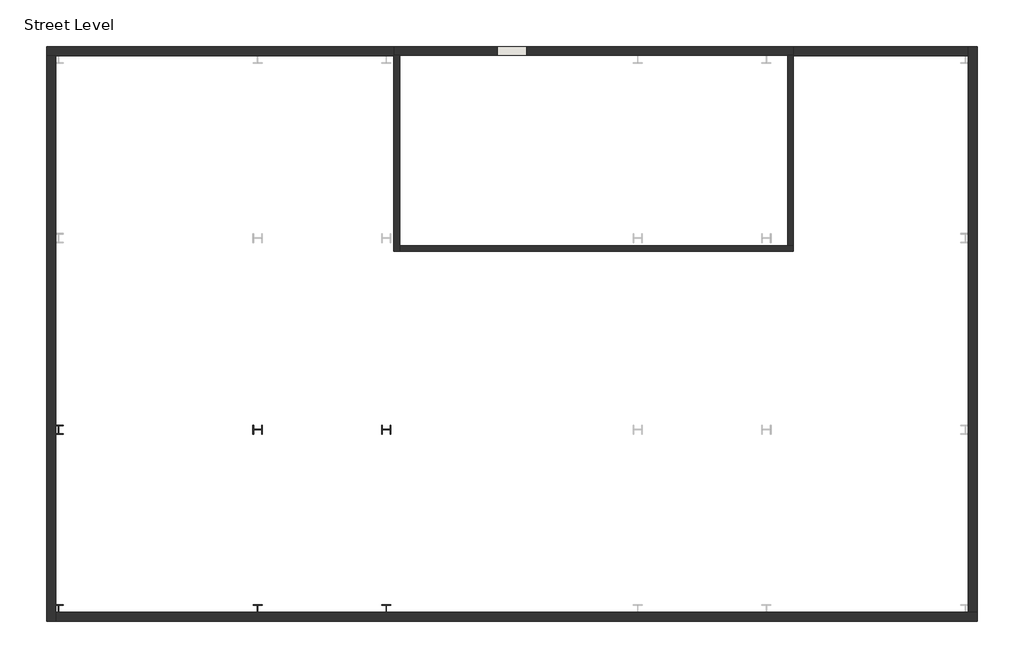
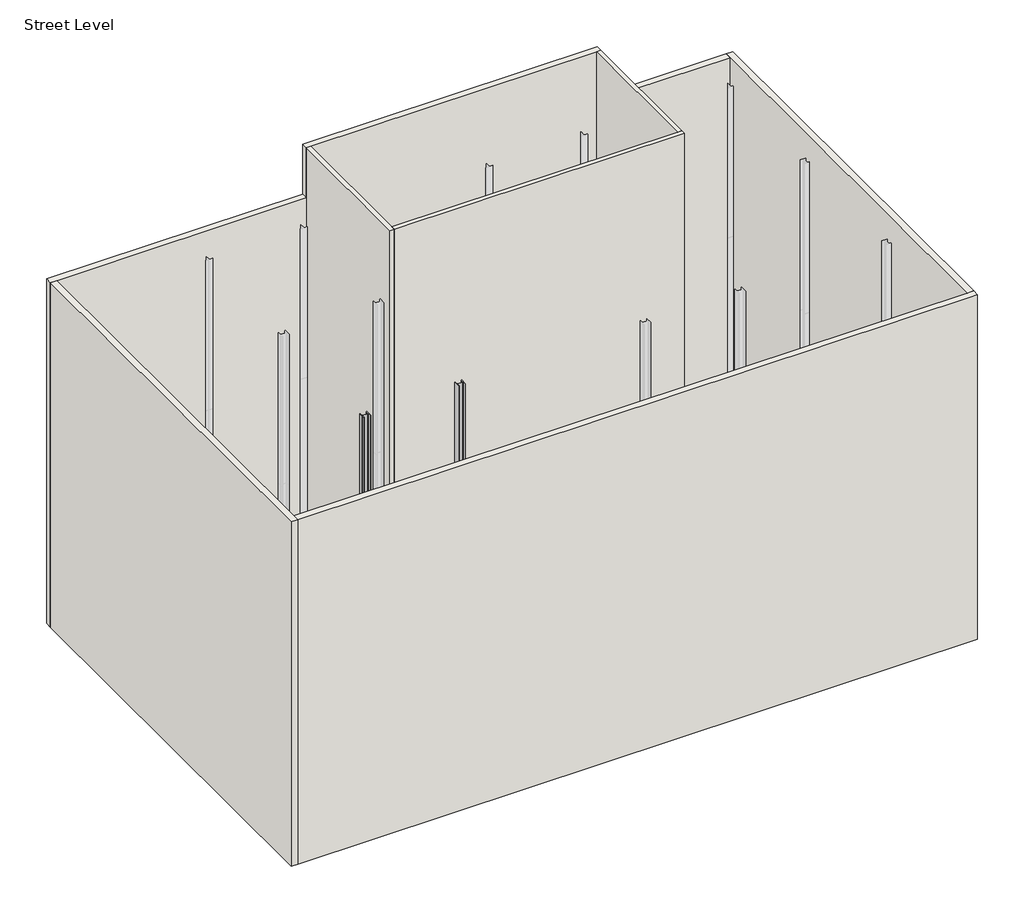
# One storey, part 1 of 3: 9 walls, 6 columns.
"""IFC4 building model written with IfcOpenShell, lengths in millimetres."""

from ifc_helpers import new_model, si_unit, point, frame, frame_2d, origin, place, context, project, spatial, polyline, circle_curve, trimmed, segment, composite_curve, outline, extrude, faceted_brep, element, save

model = new_model("IFC4")

# Units and contexts
model_context = context("Model", 3, world=origin())
ifc_project = project(units=[si_unit("LENGTHUNIT", "METRE", prefix="MILLI")], contexts=[model_context])

# Site, building, storey
site = spatial("IfcSite", under=ifc_project)
building = spatial("IfcBuilding", under=site)
storey = spatial("IfcBuildingStorey", under=building, Name="Street Level", Elevation=-914.4)

# Columns
placement = place(None, origin())
element("IfcColumn", 1, ObjectType="W-Wide Flange-Column : W12X87", at=placement, inside=storey, context=model_context, shape_type="SweptSolid", body=[
    extrude(outline(composite_curve([segment(polyline([(-9643.0622732, -3562.1684696), (-9663.6362732, -3562.1684696), (-9663.6362732, -3437.3274696)]), True, "CONTINUOUS"), segment(trimmed(circle_curve(frame_2d((-9685.9247732, -3437.3274696)), 22.2885), [point((-9663.6362732, -3437.3274696))], [point((-9685.9247732, -3415.0389696))], True, "CARTESIAN"), True, "CONTINUOUS"), segment(polyline([(-9685.9247732, -3415.0389696), (-9917.6997732, -3415.0389696)]), True, "CONTINUOUS"), segment(trimmed(circle_curve(frame_2d((-9917.6997732, -3437.3274696)), 22.2885), [point((-9917.6997732, -3415.0389696))], [point((-9939.9882732, -3437.3274696))], True, "CARTESIAN"), True, "CONTINUOUS"), segment(polyline([(-9939.9882732, -3437.3274696), (-9939.9882732, -3562.1684696), (-9960.5622732, -3562.1684696), (-9960.5622732, -3254.8284696), (-9939.9882732, -3254.8284696), (-9939.9882732, -3379.6694696)]), True, "CONTINUOUS"), segment(trimmed(circle_curve(frame_2d((-9917.6997732, -3379.6694696)), 22.2885), [point((-9939.9882732, -3379.6694696))], [point((-9917.6997732, -3401.9579696))], True, "CARTESIAN"), True, "CONTINUOUS"), segment(polyline([(-9917.6997732, -3401.9579696), (-9685.9247732, -3401.9579696)]), True, "CONTINUOUS"), segment(trimmed(circle_curve(frame_2d((-9685.9247732, -3379.6694696)), 22.2885), [point((-9685.9247732, -3401.9579696))], [point((-9663.6362732, -3379.6694696))], True, "CARTESIAN"), True, "CONTINUOUS"), segment(polyline([(-9663.6362732, -3379.6694696), (-9663.6362732, -3254.8284696), (-9643.0622732, -3254.8284696), (-9643.0622732, -3562.1684696)]), True, "CONTINUOUS")], self_intersect=False)), frame((0.0, 0.0, 7315.2), z_axis=(0.0, 0.0, 1.0), x_axis=(1.0, 0.0, 0.0)), (0.0, 0.0, 1.0), 7315.2),
    extrude(outline(composite_curve([segment(polyline([(-9643.0622732, -3562.1684696), (-9663.6362732, -3562.1684696), (-9663.6362732, -3437.3274696)]), True, "CONTINUOUS"), segment(trimmed(circle_curve(frame_2d((-9685.9247732, -3437.3274696)), 22.2885), [point((-9663.6362732, -3437.3274696))], [point((-9685.9247732, -3415.0389696))], True, "CARTESIAN"), True, "CONTINUOUS"), segment(polyline([(-9685.9247732, -3415.0389696), (-9917.6997732, -3415.0389696)]), True, "CONTINUOUS"), segment(trimmed(circle_curve(frame_2d((-9917.6997732, -3437.3274696)), 22.2885), [point((-9917.6997732, -3415.0389696))], [point((-9939.9882732, -3437.3274696))], True, "CARTESIAN"), True, "CONTINUOUS"), segment(polyline([(-9939.9882732, -3437.3274696), (-9939.9882732, -3562.1684696), (-9960.5622732, -3562.1684696), (-9960.5622732, -3254.8284696), (-9939.9882732, -3254.8284696), (-9939.9882732, -3379.6694696)]), True, "CONTINUOUS"), segment(trimmed(circle_curve(frame_2d((-9917.6997732, -3379.6694696)), 22.2885), [point((-9939.9882732, -3379.6694696))], [point((-9917.6997732, -3401.9579696))], True, "CARTESIAN"), True, "CONTINUOUS"), segment(polyline([(-9917.6997732, -3401.9579696), (-9685.9247732, -3401.9579696)]), True, "CONTINUOUS"), segment(trimmed(circle_curve(frame_2d((-9685.9247732, -3379.6694696)), 22.2885), [point((-9685.9247732, -3401.9579696))], [point((-9663.6362732, -3379.6694696))], True, "CARTESIAN"), True, "CONTINUOUS"), segment(polyline([(-9663.6362732, -3379.6694696), (-9663.6362732, -3254.8284696), (-9643.0622732, -3254.8284696), (-9643.0622732, -3562.1684696)]), True, "CONTINUOUS")], self_intersect=False)), frame((0.0, 0.0, -914.4), z_axis=(0.0, 0.0, 1.0), x_axis=(1.0, 0.0, 0.0)), (0.0, 0.0, 1.0), 8229.6),
])
element("IfcColumn", 2, ObjectType="W-Wide Flange-Column : W12X87", at=placement, inside=storey, context=model_context, shape_type="SweptSolid", body=[
    extrude(outline(composite_curve([segment(polyline([(-5274.2622732, -3562.1684696), (-5294.8362732, -3562.1684696), (-5294.8362732, -3437.3274696)]), True, "CONTINUOUS"), segment(trimmed(circle_curve(frame_2d((-5317.1247732, -3437.3274696)), 22.2885), [point((-5294.8362732, -3437.3274696))], [point((-5317.1247732, -3415.0389696))], True, "CARTESIAN"), True, "CONTINUOUS"), segment(polyline([(-5317.1247732, -3415.0389696), (-5548.8997732, -3415.0389696)]), True, "CONTINUOUS"), segment(trimmed(circle_curve(frame_2d((-5548.8997732, -3437.3274696)), 22.2885), [point((-5548.8997732, -3415.0389696))], [point((-5571.1882732, -3437.3274696))], True, "CARTESIAN"), True, "CONTINUOUS"), segment(polyline([(-5571.1882732, -3437.3274696), (-5571.1882732, -3562.1684696), (-5591.7622732, -3562.1684696), (-5591.7622732, -3254.8284696), (-5571.1882732, -3254.8284696), (-5571.1882732, -3379.6694696)]), True, "CONTINUOUS"), segment(trimmed(circle_curve(frame_2d((-5548.8997732, -3379.6694696)), 22.2885), [point((-5571.1882732, -3379.6694696))], [point((-5548.8997732, -3401.9579696))], True, "CARTESIAN"), True, "CONTINUOUS"), segment(polyline([(-5548.8997732, -3401.9579696), (-5317.1247732, -3401.9579696)]), True, "CONTINUOUS"), segment(trimmed(circle_curve(frame_2d((-5317.1247732, -3379.6694696)), 22.2885), [point((-5317.1247732, -3401.9579696))], [point((-5294.8362732, -3379.6694696))], True, "CARTESIAN"), True, "CONTINUOUS"), segment(polyline([(-5294.8362732, -3379.6694696), (-5294.8362732, -3254.8284696), (-5274.2622732, -3254.8284696), (-5274.2622732, -3562.1684696)]), True, "CONTINUOUS")], self_intersect=False)), frame((0.0, 0.0, 7315.2), z_axis=(0.0, 0.0, 1.0), x_axis=(1.0, 0.0, 0.0)), (0.0, 0.0, 1.0), 7315.2),
    extrude(outline(composite_curve([segment(polyline([(-5274.2622732, -3562.1684696), (-5294.8362732, -3562.1684696), (-5294.8362732, -3437.3274696)]), True, "CONTINUOUS"), segment(trimmed(circle_curve(frame_2d((-5317.1247732, -3437.3274696)), 22.2885), [point((-5294.8362732, -3437.3274696))], [point((-5317.1247732, -3415.0389696))], True, "CARTESIAN"), True, "CONTINUOUS"), segment(polyline([(-5317.1247732, -3415.0389696), (-5548.8997732, -3415.0389696)]), True, "CONTINUOUS"), segment(trimmed(circle_curve(frame_2d((-5548.8997732, -3437.3274696)), 22.2885), [point((-5548.8997732, -3415.0389696))], [point((-5571.1882732, -3437.3274696))], True, "CARTESIAN"), True, "CONTINUOUS"), segment(polyline([(-5571.1882732, -3437.3274696), (-5571.1882732, -3562.1684696), (-5591.7622732, -3562.1684696), (-5591.7622732, -3254.8284696), (-5571.1882732, -3254.8284696), (-5571.1882732, -3379.6694696)]), True, "CONTINUOUS"), segment(trimmed(circle_curve(frame_2d((-5548.8997732, -3379.6694696)), 22.2885), [point((-5571.1882732, -3379.6694696))], [point((-5548.8997732, -3401.9579696))], True, "CARTESIAN"), True, "CONTINUOUS"), segment(polyline([(-5548.8997732, -3401.9579696), (-5317.1247732, -3401.9579696)]), True, "CONTINUOUS"), segment(trimmed(circle_curve(frame_2d((-5317.1247732, -3379.6694696)), 22.2885), [point((-5317.1247732, -3401.9579696))], [point((-5294.8362732, -3379.6694696))], True, "CARTESIAN"), True, "CONTINUOUS"), segment(polyline([(-5294.8362732, -3379.6694696), (-5294.8362732, -3254.8284696), (-5274.2622732, -3254.8284696), (-5274.2622732, -3562.1684696)]), True, "CONTINUOUS")], self_intersect=False)), frame((0.0, 0.0, -914.4), z_axis=(0.0, 0.0, 1.0), x_axis=(1.0, 0.0, 0.0)), (0.0, 0.0, 1.0), 8229.6),
])
element("IfcColumn", 3, ObjectType="W-Wide Flange-Column : W12X87", at=placement, inside=storey, context=model_context, shape_type="SweptSolid", body=[
    extrude(outline(composite_curve([segment(polyline([(-5279.3422732, -9345.7484696), (-5279.3422732, -9366.3224696), (-5404.1832732, -9366.3224696)]), True, "CONTINUOUS"), segment(trimmed(circle_curve(frame_2d((-5404.1832732, -9388.6109696)), 22.2885), [point((-5404.1832732, -9366.3224696))], [point((-5426.4717732, -9388.6109696))], True, "CARTESIAN"), True, "CONTINUOUS"), segment(polyline([(-5426.4717732, -9388.6109696), (-5426.4717732, -9620.3859696)]), True, "CONTINUOUS"), segment(trimmed(circle_curve(frame_2d((-5404.1832732, -9620.3859696)), 22.2885), [point((-5426.4717732, -9620.3859696))], [point((-5404.1832732, -9642.6744696))], True, "CARTESIAN"), True, "CONTINUOUS"), segment(polyline([(-5404.1832732, -9642.6744696), (-5279.3422732, -9642.6744696), (-5279.3422732, -9663.2484696), (-5586.6822732, -9663.2484696), (-5586.6822732, -9642.6744696), (-5461.8412732, -9642.6744696)]), True, "CONTINUOUS"), segment(trimmed(circle_curve(frame_2d((-5461.8412732, -9620.3859696)), 22.2885), [point((-5461.8412732, -9642.6744696))], [point((-5439.5527732, -9620.3859696))], True, "CARTESIAN"), True, "CONTINUOUS"), segment(polyline([(-5439.5527732, -9620.3859696), (-5439.5527732, -9388.6109696)]), True, "CONTINUOUS"), segment(trimmed(circle_curve(frame_2d((-5461.8412732, -9388.6109696)), 22.2885), [point((-5439.5527732, -9388.6109696))], [point((-5461.8412732, -9366.3224696))], True, "CARTESIAN"), True, "CONTINUOUS"), segment(polyline([(-5461.8412732, -9366.3224696), (-5586.6822732, -9366.3224696), (-5586.6822732, -9345.7484696), (-5279.3422732, -9345.7484696)]), True, "CONTINUOUS")], self_intersect=False)), frame((0.0, 0.0, 7315.2), z_axis=(0.0, 0.0, 1.0), x_axis=(1.0, 0.0, 0.0)), (0.0, 0.0, 1.0), 7315.2),
    extrude(outline(composite_curve([segment(polyline([(-5279.3422732, -9345.7484696), (-5279.3422732, -9366.3224696), (-5404.1832732, -9366.3224696)]), True, "CONTINUOUS"), segment(trimmed(circle_curve(frame_2d((-5404.1832732, -9388.6109696)), 22.2885), [point((-5404.1832732, -9366.3224696))], [point((-5426.4717732, -9388.6109696))], True, "CARTESIAN"), True, "CONTINUOUS"), segment(polyline([(-5426.4717732, -9388.6109696), (-5426.4717732, -9620.3859696)]), True, "CONTINUOUS"), segment(trimmed(circle_curve(frame_2d((-5404.1832732, -9620.3859696)), 22.2885), [point((-5426.4717732, -9620.3859696))], [point((-5404.1832732, -9642.6744696))], True, "CARTESIAN"), True, "CONTINUOUS"), segment(polyline([(-5404.1832732, -9642.6744696), (-5279.3422732, -9642.6744696), (-5279.3422732, -9663.2484696), (-5586.6822732, -9663.2484696), (-5586.6822732, -9642.6744696), (-5461.8412732, -9642.6744696)]), True, "CONTINUOUS"), segment(trimmed(circle_curve(frame_2d((-5461.8412732, -9620.3859696)), 22.2885), [point((-5461.8412732, -9642.6744696))], [point((-5439.5527732, -9620.3859696))], True, "CARTESIAN"), True, "CONTINUOUS"), segment(polyline([(-5439.5527732, -9620.3859696), (-5439.5527732, -9388.6109696)]), True, "CONTINUOUS"), segment(trimmed(circle_curve(frame_2d((-5461.8412732, -9388.6109696)), 22.2885), [point((-5439.5527732, -9388.6109696))], [point((-5461.8412732, -9366.3224696))], True, "CARTESIAN"), True, "CONTINUOUS"), segment(polyline([(-5461.8412732, -9366.3224696), (-5586.6822732, -9366.3224696), (-5586.6822732, -9345.7484696), (-5279.3422732, -9345.7484696)]), True, "CONTINUOUS")], self_intersect=False)), frame((0.0, 0.0, -914.4), z_axis=(0.0, 0.0, 1.0), x_axis=(1.0, 0.0, 0.0)), (0.0, 0.0, 1.0), 8229.6),
])
element("IfcColumn", 4, ObjectType="W-Wide Flange-Column : W12X87", at=placement, inside=storey, context=model_context, shape_type="SweptSolid", body=[
    extrude(outline(composite_curve([segment(polyline([(-9648.1422732, -9345.7484696), (-9648.1422732, -9366.3224696), (-9772.9832732, -9366.3224696)]), True, "CONTINUOUS"), segment(trimmed(circle_curve(frame_2d((-9772.9832732, -9388.6109696)), 22.2885), [point((-9772.9832732, -9366.3224696))], [point((-9795.2717732, -9388.6109696))], True, "CARTESIAN"), True, "CONTINUOUS"), segment(polyline([(-9795.2717732, -9388.6109696), (-9795.2717732, -9620.3859696)]), True, "CONTINUOUS"), segment(trimmed(circle_curve(frame_2d((-9772.9832732, -9620.3859696)), 22.2885), [point((-9795.2717732, -9620.3859696))], [point((-9772.9832732, -9642.6744696))], True, "CARTESIAN"), True, "CONTINUOUS"), segment(polyline([(-9772.9832732, -9642.6744696), (-9648.1422732, -9642.6744696), (-9648.1422732, -9663.2484696), (-9955.4822732, -9663.2484696), (-9955.4822732, -9642.6744696), (-9830.6412732, -9642.6744696)]), True, "CONTINUOUS"), segment(trimmed(circle_curve(frame_2d((-9830.6412732, -9620.3859696)), 22.2885), [point((-9830.6412732, -9642.6744696))], [point((-9808.3527732, -9620.3859696))], True, "CARTESIAN"), True, "CONTINUOUS"), segment(polyline([(-9808.3527732, -9620.3859696), (-9808.3527732, -9388.6109696)]), True, "CONTINUOUS"), segment(trimmed(circle_curve(frame_2d((-9830.6412732, -9388.6109696)), 22.2885), [point((-9808.3527732, -9388.6109696))], [point((-9830.6412732, -9366.3224696))], True, "CARTESIAN"), True, "CONTINUOUS"), segment(polyline([(-9830.6412732, -9366.3224696), (-9955.4822732, -9366.3224696), (-9955.4822732, -9345.7484696), (-9648.1422732, -9345.7484696)]), True, "CONTINUOUS")], self_intersect=False)), frame((0.0, 0.0, 7315.2), z_axis=(0.0, 0.0, 1.0), x_axis=(1.0, 0.0, 0.0)), (0.0, 0.0, 1.0), 7315.2),
    extrude(outline(composite_curve([segment(polyline([(-9648.1422732, -9345.7484696), (-9648.1422732, -9366.3224696), (-9772.9832732, -9366.3224696)]), True, "CONTINUOUS"), segment(trimmed(circle_curve(frame_2d((-9772.9832732, -9388.6109696)), 22.2885), [point((-9772.9832732, -9366.3224696))], [point((-9795.2717732, -9388.6109696))], True, "CARTESIAN"), True, "CONTINUOUS"), segment(polyline([(-9795.2717732, -9388.6109696), (-9795.2717732, -9620.3859696)]), True, "CONTINUOUS"), segment(trimmed(circle_curve(frame_2d((-9772.9832732, -9620.3859696)), 22.2885), [point((-9795.2717732, -9620.3859696))], [point((-9772.9832732, -9642.6744696))], True, "CARTESIAN"), True, "CONTINUOUS"), segment(polyline([(-9772.9832732, -9642.6744696), (-9648.1422732, -9642.6744696), (-9648.1422732, -9663.2484696), (-9955.4822732, -9663.2484696), (-9955.4822732, -9642.6744696), (-9830.6412732, -9642.6744696)]), True, "CONTINUOUS"), segment(trimmed(circle_curve(frame_2d((-9830.6412732, -9620.3859696)), 22.2885), [point((-9830.6412732, -9642.6744696))], [point((-9808.3527732, -9620.3859696))], True, "CARTESIAN"), True, "CONTINUOUS"), segment(polyline([(-9808.3527732, -9620.3859696), (-9808.3527732, -9388.6109696)]), True, "CONTINUOUS"), segment(trimmed(circle_curve(frame_2d((-9830.6412732, -9388.6109696)), 22.2885), [point((-9808.3527732, -9388.6109696))], [point((-9830.6412732, -9366.3224696))], True, "CARTESIAN"), True, "CONTINUOUS"), segment(polyline([(-9830.6412732, -9366.3224696), (-9955.4822732, -9366.3224696), (-9955.4822732, -9345.7484696), (-9648.1422732, -9345.7484696)]), True, "CONTINUOUS")], self_intersect=False)), frame((0.0, 0.0, -914.4), z_axis=(0.0, 0.0, 1.0), x_axis=(1.0, 0.0, 0.0)), (0.0, 0.0, 1.0), 8229.6),
])
element("IfcColumn", 5, ObjectType="W-Wide Flange-Column : W12X87", at=placement, inside=storey, context=model_context, shape_type="SweptSolid", body=[
    extrude(outline(composite_curve([segment(polyline([(-16404.5422732, -9345.7484696), (-16404.5422732, -9366.3224696), (-16529.3832732, -9366.3224696)]), True, "CONTINUOUS"), segment(trimmed(circle_curve(frame_2d((-16529.3832732, -9388.6109696)), 22.2885), [point((-16529.3832732, -9366.3224696))], [point((-16551.6717732, -9388.6109696))], True, "CARTESIAN"), True, "CONTINUOUS"), segment(polyline([(-16551.6717732, -9388.6109696), (-16551.6717732, -9620.3859696)]), True, "CONTINUOUS"), segment(trimmed(circle_curve(frame_2d((-16529.3832732, -9620.3859696)), 22.2885), [point((-16551.6717732, -9620.3859696))], [point((-16529.3832732, -9642.6744696))], True, "CARTESIAN"), True, "CONTINUOUS"), segment(polyline([(-16529.3832732, -9642.6744696), (-16404.5422732, -9642.6744696), (-16404.5422732, -9663.2484696), (-16711.8822732, -9663.2484696), (-16711.8822732, -9642.6744696), (-16587.0412732, -9642.6744696)]), True, "CONTINUOUS"), segment(trimmed(circle_curve(frame_2d((-16587.0412732, -9620.3859696)), 22.2885), [point((-16587.0412732, -9642.6744696))], [point((-16564.7527732, -9620.3859696))], True, "CARTESIAN"), True, "CONTINUOUS"), segment(polyline([(-16564.7527732, -9620.3859696), (-16564.7527732, -9388.6109696)]), True, "CONTINUOUS"), segment(trimmed(circle_curve(frame_2d((-16587.0412732, -9388.6109696)), 22.2885), [point((-16564.7527732, -9388.6109696))], [point((-16587.0412732, -9366.3224696))], True, "CARTESIAN"), True, "CONTINUOUS"), segment(polyline([(-16587.0412732, -9366.3224696), (-16711.8822732, -9366.3224696), (-16711.8822732, -9345.7484696), (-16404.5422732, -9345.7484696)]), True, "CONTINUOUS")], self_intersect=False)), frame((0.0, 0.0, 7315.2), z_axis=(0.0, 0.0, 1.0), x_axis=(1.0, 0.0, 0.0)), (0.0, 0.0, 1.0), 7315.2),
    extrude(outline(composite_curve([segment(polyline([(-16404.5422732, -9345.7484696), (-16404.5422732, -9366.3224696), (-16529.3832732, -9366.3224696)]), True, "CONTINUOUS"), segment(trimmed(circle_curve(frame_2d((-16529.3832732, -9388.6109696)), 22.2885), [point((-16529.3832732, -9366.3224696))], [point((-16551.6717732, -9388.6109696))], True, "CARTESIAN"), True, "CONTINUOUS"), segment(polyline([(-16551.6717732, -9388.6109696), (-16551.6717732, -9620.3859696)]), True, "CONTINUOUS"), segment(trimmed(circle_curve(frame_2d((-16529.3832732, -9620.3859696)), 22.2885), [point((-16551.6717732, -9620.3859696))], [point((-16529.3832732, -9642.6744696))], True, "CARTESIAN"), True, "CONTINUOUS"), segment(polyline([(-16529.3832732, -9642.6744696), (-16404.5422732, -9642.6744696), (-16404.5422732, -9663.2484696), (-16711.8822732, -9663.2484696), (-16711.8822732, -9642.6744696), (-16587.0412732, -9642.6744696)]), True, "CONTINUOUS"), segment(trimmed(circle_curve(frame_2d((-16587.0412732, -9620.3859696)), 22.2885), [point((-16587.0412732, -9642.6744696))], [point((-16564.7527732, -9620.3859696))], True, "CARTESIAN"), True, "CONTINUOUS"), segment(polyline([(-16564.7527732, -9620.3859696), (-16564.7527732, -9388.6109696)]), True, "CONTINUOUS"), segment(trimmed(circle_curve(frame_2d((-16587.0412732, -9388.6109696)), 22.2885), [point((-16564.7527732, -9388.6109696))], [point((-16587.0412732, -9366.3224696))], True, "CARTESIAN"), True, "CONTINUOUS"), segment(polyline([(-16587.0412732, -9366.3224696), (-16711.8822732, -9366.3224696), (-16711.8822732, -9345.7484696), (-16404.5422732, -9345.7484696)]), True, "CONTINUOUS")], self_intersect=False)), frame((0.0, 0.0, -914.4), z_axis=(0.0, 0.0, 1.0), x_axis=(1.0, 0.0, 0.0)), (0.0, 0.0, 1.0), 8229.6),
])
element("IfcColumn", 6, ObjectType="W-Wide Flange-Column : W12X87", at=placement, inside=storey, context=model_context, shape_type="SweptSolid", body=[
    extrude(outline(composite_curve([segment(polyline([(-16404.5422732, -3249.7484696), (-16404.5422732, -3270.3224696), (-16529.3832732, -3270.3224696)]), True, "CONTINUOUS"), segment(trimmed(circle_curve(frame_2d((-16529.3832732, -3292.6109696)), 22.2885), [point((-16529.3832732, -3270.3224696))], [point((-16551.6717732, -3292.6109696))], True, "CARTESIAN"), True, "CONTINUOUS"), segment(polyline([(-16551.6717732, -3292.6109696), (-16551.6717732, -3524.3859696)]), True, "CONTINUOUS"), segment(trimmed(circle_curve(frame_2d((-16529.3832732, -3524.3859696)), 22.2885), [point((-16551.6717732, -3524.3859696))], [point((-16529.3832732, -3546.6744696))], True, "CARTESIAN"), True, "CONTINUOUS"), segment(polyline([(-16529.3832732, -3546.6744696), (-16404.5422732, -3546.6744696), (-16404.5422732, -3567.2484696), (-16711.8822732, -3567.2484696), (-16711.8822732, -3546.6744696), (-16587.0412732, -3546.6744696)]), True, "CONTINUOUS"), segment(trimmed(circle_curve(frame_2d((-16587.0412732, -3524.3859696)), 22.2885), [point((-16587.0412732, -3546.6744696))], [point((-16564.7527732, -3524.3859696))], True, "CARTESIAN"), True, "CONTINUOUS"), segment(polyline([(-16564.7527732, -3524.3859696), (-16564.7527732, -3292.6109696)]), True, "CONTINUOUS"), segment(trimmed(circle_curve(frame_2d((-16587.0412732, -3292.6109696)), 22.2885), [point((-16564.7527732, -3292.6109696))], [point((-16587.0412732, -3270.3224696))], True, "CARTESIAN"), True, "CONTINUOUS"), segment(polyline([(-16587.0412732, -3270.3224696), (-16711.8822732, -3270.3224696), (-16711.8822732, -3249.7484696), (-16404.5422732, -3249.7484696)]), True, "CONTINUOUS")], self_intersect=False)), frame((0.0, 0.0, 7315.2), z_axis=(0.0, 0.0, 1.0), x_axis=(1.0, 0.0, 0.0)), (0.0, 0.0, 1.0), 7315.2),
    extrude(outline(composite_curve([segment(polyline([(-16404.5422732, -3249.7484696), (-16404.5422732, -3270.3224696), (-16529.3832732, -3270.3224696)]), True, "CONTINUOUS"), segment(trimmed(circle_curve(frame_2d((-16529.3832732, -3292.6109696)), 22.2885), [point((-16529.3832732, -3270.3224696))], [point((-16551.6717732, -3292.6109696))], True, "CARTESIAN"), True, "CONTINUOUS"), segment(polyline([(-16551.6717732, -3292.6109696), (-16551.6717732, -3524.3859696)]), True, "CONTINUOUS"), segment(trimmed(circle_curve(frame_2d((-16529.3832732, -3524.3859696)), 22.2885), [point((-16551.6717732, -3524.3859696))], [point((-16529.3832732, -3546.6744696))], True, "CARTESIAN"), True, "CONTINUOUS"), segment(polyline([(-16529.3832732, -3546.6744696), (-16404.5422732, -3546.6744696), (-16404.5422732, -3567.2484696), (-16711.8822732, -3567.2484696), (-16711.8822732, -3546.6744696), (-16587.0412732, -3546.6744696)]), True, "CONTINUOUS"), segment(trimmed(circle_curve(frame_2d((-16587.0412732, -3524.3859696)), 22.2885), [point((-16587.0412732, -3546.6744696))], [point((-16564.7527732, -3524.3859696))], True, "CARTESIAN"), True, "CONTINUOUS"), segment(polyline([(-16564.7527732, -3524.3859696), (-16564.7527732, -3292.6109696)]), True, "CONTINUOUS"), segment(trimmed(circle_curve(frame_2d((-16587.0412732, -3292.6109696)), 22.2885), [point((-16564.7527732, -3292.6109696))], [point((-16587.0412732, -3270.3224696))], True, "CARTESIAN"), True, "CONTINUOUS"), segment(polyline([(-16587.0412732, -3270.3224696), (-16711.8822732, -3270.3224696), (-16711.8822732, -3249.7484696), (-16404.5422732, -3249.7484696)]), True, "CONTINUOUS")], self_intersect=False)), frame((0.0, 0.0, -914.4), z_axis=(0.0, 0.0, 1.0), x_axis=(1.0, 0.0, 0.0)), (0.0, 0.0, 1.0), 8229.6),
])

# Walls
element("IfcWall", 7, ObjectType="Generic - 12\"", at=placement, inside=storey, context=model_context, shape_type="Brep", body=[
    faceted_brep([(-16964.6122732, 9291.5015304, -914.4), (-16659.8122732, 9291.5015304, -914.4), (-5174.2497732, 9291.5015304, -914.4), (-5174.2497732, 9291.5015304, 0.0), (-5174.2497732, 9291.5015304, 3657.6), (-5174.2497732, 9291.5015304, 7315.2), (-5174.2497732, 9291.5015304, 10972.8), (-5174.2497732, 9291.5015304, 14630.4), (-5174.2497732, 9291.5015304, 15849.6), (-16659.8122732, 9291.5015304, 15849.6), (-16964.6122732, 9291.5015304, 15849.6), (-16964.6122732, 9596.3015304, -914.4), (-16964.6122732, 9596.3015304, 15849.6), (-5174.2497732, 9596.3015304, 15849.6), (-5174.2497732, 9596.3015304, -914.4)], [[[0, 1, 2, 3, 4, 5, 6, 7, 8, 9, 10]], [[11, 12, 13, 14]], [[2, 1, 0, 11, 14]], [[10, 9, 8, 13, 12]], [[0, 10, 12, 11]], [[8, 7, 6, 5, 4, 3, 2, 14, 13]]]),
])
element("IfcWall", 8, ObjectType="Generic - 12\"", at=placement, inside=storey, context=model_context, shape_type="Brep", body=[
    faceted_brep([(-16659.8122732, -9910.8984696, -914.4), (-16659.8122732, -9606.0984696, -914.4), (-16659.8122732, 9291.5015304, -914.4), (-16659.8122732, 9291.5015304, 0.0), (-16659.8122732, 9291.5015304, 3657.6), (-16659.8122732, 9291.5015304, 7010.4), (-16659.8122732, 9291.5015304, 7315.2), (-16659.8122732, 9291.5015304, 10972.8), (-16659.8122732, 9291.5015304, 14630.4), (-16659.8122732, 9291.5015304, 15849.6), (-16659.8122732, -9606.0984696, 15849.6), (-16659.8122732, -9910.8984696, 15849.6), (-16964.6122732, -9910.8984696, -914.4), (-16964.6122732, -9910.8984696, 15849.6), (-16964.6122732, 9291.5015304, 15849.6), (-16964.6122732, 9291.5015304, -914.4)], [[[0, 1, 2, 3, 4, 5, 6, 7, 8, 9, 10, 11]], [[12, 13, 14, 15]], [[2, 1, 0, 12, 15]], [[11, 10, 9, 14, 13]], [[0, 11, 13, 12]], [[9, 8, 7, 6, 5, 4, 3, 2, 15, 14]]]),
])
element("IfcWall", 9, ObjectType="Generic - 12\"", at=placement, inside=storey, context=model_context, shape_type="Brep", body=[
    faceted_brep([(14632.9877268, -9606.0984696, -914.4), (14328.1877268, -9606.0984696, -914.4), (-16659.8122732, -9606.0984696, -914.4), (-16659.8122732, -9606.0984696, 0.0), (-16659.8122732, -9606.0984696, 3657.6), (-16659.8122732, -9606.0984696, 7010.4), (-16659.8122732, -9606.0984696, 7315.2), (-16659.8122732, -9606.0984696, 10972.8), (-16659.8122732, -9606.0984696, 14630.4), (-16659.8122732, -9606.0984696, 15849.6), (14328.1877268, -9606.0984696, 15849.6), (14632.9877268, -9606.0984696, 15849.6), (14632.9877268, -9910.8984696, -914.4), (14632.9877268, -9910.8984696, 15849.6), (-16659.8122732, -9910.8984696, 15849.6), (-16659.8122732, -9910.8984696, -914.4)], [[[0, 1, 2, 3, 4, 5, 6, 7, 8, 9, 10, 11]], [[12, 13, 14, 15]], [[2, 1, 0, 12, 15]], [[11, 10, 9, 14, 13]], [[0, 11, 13, 12]], [[9, 8, 7, 6, 5, 4, 3, 2, 15, 14]]]),
])
element("IfcWall", 10, ObjectType="Generic - 12\"", at=placement, inside=storey, context=model_context, shape_type="Brep", body=[
    faceted_brep([(14328.1877268, 9596.3015304, -914.4), (14328.1877268, 9291.5015304, -914.4), (14328.1877268, -9606.0984696, -914.4), (14328.1877268, -9606.0984696, 0.0), (14328.1877268, -9606.0984696, 3657.6), (14328.1877268, -9606.0984696, 7010.4), (14328.1877268, -9606.0984696, 7315.2), (14328.1877268, -9606.0984696, 10972.8), (14328.1877268, -9606.0984696, 14630.4), (14328.1877268, -9606.0984696, 15849.6), (14328.1877268, 9291.5015304, 15849.6), (14328.1877268, 9596.3015304, 15849.6), (14632.9877268, 9596.3015304, -914.4), (14632.9877268, 9596.3015304, 15849.6), (14632.9877268, -9606.0984696, 15849.6), (14632.9877268, -9606.0984696, -914.4)], [[[0, 1, 2, 3, 4, 5, 6, 7, 8, 9, 10, 11]], [[12, 13, 14, 15]], [[2, 1, 0, 12, 15]], [[11, 10, 9, 14, 13]], [[0, 11, 13, 12]], [[9, 8, 7, 6, 5, 4, 3, 2, 15, 14]]]),
])
element("IfcWall", 11, ObjectType="Generic - 12\"", at=placement, inside=storey, context=model_context, shape_type="SweptSolid", body=[
    extrude(outline(polyline([(14328.1877268, 9291.5015304), (8379.8252268, 9291.5015304), (8379.8252268, 9596.3015304), (14328.1877268, 9596.3015304), (14328.1877268, 9291.5015304)])), frame((0.0, 0.0, -914.4), z_axis=(0.0, 0.0, 1.0), x_axis=(1.0, 0.0, 0.0)), (0.0, 0.0, 1.0), 16764.0),
])
element("IfcWall", 12, ObjectType="Generic - 12\" Masonry", at=placement, inside=storey, context=model_context, shape_type="Brep", body=[
    faceted_brep([(-5174.2497732, 9301.0265304, 18288.0), (-5174.2497732, 9301.0265304, -914.4), (-4980.5747732, 9301.0265304, -914.4), (8186.1502268, 9301.0265304, -914.4), (8379.8252268, 9301.0265304, -914.4), (8379.8252268, 9301.0265304, 18288.0), (8186.1502268, 9301.0265304, 18288.0), (-4980.5747732, 9301.0265304, 18288.0), (-1673.8122732, 9301.0265304, 0.0), (-1673.8122732, 9301.0265304, 2235.2), (-657.8122732, 9301.0265304, 2235.2), (-657.8122732, 9301.0265304, 0.0), (-5174.2497732, 9596.3015304, -914.4), (-5174.2497732, 9596.3015304, 18288.0), (8379.8252268, 9596.3015304, 18288.0), (8379.8252268, 9596.3015304, -914.4), (-1673.8122732, 9596.3015304, 0.0), (-657.8122732, 9596.3015304, 0.0), (-657.8122732, 9596.3015304, 2235.2), (-1673.8122732, 9596.3015304, 2235.2)], [[[0, 1, 2, 3, 4, 5, 6, 7], [8, 9, 10, 11]], [[12, 13, 14, 15], [16, 17, 18, 19]], [[4, 3, 2, 1, 12, 15]], [[0, 7, 6, 5, 14, 13]], [[8, 11, 17, 16]], [[11, 10, 18, 17]], [[10, 9, 19, 18]], [[9, 8, 16, 19]], [[0, 13, 12, 1]], [[4, 15, 14, 5]]]),
])
element("IfcWall", 13, ObjectType="Generic - 8\" Masonry", at=placement, inside=storey, context=model_context, shape_type="Brep", body=[
    faceted_brep([(-5174.2497732, 9301.0265304, 18288.0), (-5174.2497732, 9301.0265304, 14630.4), (-5174.2497732, 9301.0265304, 10972.8), (-5174.2497732, 9301.0265304, 7315.2), (-5174.2497732, 9301.0265304, 3657.6), (-5174.2497732, 9301.0265304, 0.0), (-5174.2497732, 9301.0265304, -914.4), (-5174.2497732, 2641.4640304, -914.4), (-5174.2497732, 2641.4640304, 18288.0), (-4980.5747732, 9301.0265304, -914.4), (-4980.5747732, 9301.0265304, 18288.0), (-4980.5747732, 2835.1390304, 18288.0), (-4980.5747732, 2641.4640304, 18288.0), (-4980.5747732, 2641.4640304, -914.4), (-4980.5747732, 2835.1390304, -914.4)], [[[0, 1, 2, 3, 4, 5, 6, 7, 8]], [[9, 10, 11, 12, 13, 14]], [[7, 6, 9, 14, 13]], [[0, 8, 12, 11, 10]], [[8, 7, 13, 12]], [[0, 10, 9, 6, 5, 4, 3, 2, 1]]]),
])
element("IfcWall", 14, ObjectType="Generic - 8\" Masonry", at=placement, inside=storey, context=model_context, shape_type="Brep", body=[
    faceted_brep([(8379.8252268, 2835.1390304, -914.4), (8186.1502268, 2835.1390304, -914.4), (-4980.5747732, 2835.1390304, -914.4), (-4980.5747732, 2835.1390304, 18288.0), (8186.1502268, 2835.1390304, 18288.0), (8379.8252268, 2835.1390304, 18288.0), (8379.8252268, 2641.4640304, -914.4), (8379.8252268, 2641.4640304, 18288.0), (-4980.5747732, 2641.4640304, 18288.0), (-4980.5747732, 2641.4640304, -914.4)], [[[0, 1, 2, 3, 4, 5]], [[6, 7, 8, 9]], [[2, 1, 0, 6, 9]], [[5, 4, 3, 8, 7]], [[3, 2, 9, 8]], [[0, 5, 7, 6]]]),
])
element("IfcWall", 15, ObjectType="Generic - 8\" Masonry", at=placement, inside=storey, context=model_context, shape_type="SweptSolid", body=[
    extrude(outline(polyline([(8186.1502268, 2835.1390304), (8186.1502268, 9301.0265304), (8379.8252268, 9301.0265304), (8379.8252268, 2835.1390304), (8186.1502268, 2835.1390304)])), frame((0.0, 0.0, -914.4), z_axis=(0.0, 0.0, 1.0), x_axis=(1.0, 0.0, 0.0)), (0.0, 0.0, 1.0), 19202.4),
])

save(model, "model.ifc")

# Revit data of these elements
# Type "W-Wide Flange-Column : W12X87"
#   Assembly Code = "B10"
#   W = 87
#   bf = 1' - 0.1"
#   d = 1' - 0 1/2"
#   k = 0' - 1 11/16"
#   kr = 0' - 0.8775"
#   tf = 0' - 0.81"
#   tw = 0' - 0.515"
#   A = 0.177778 SF
#   Structural Material [instance default] = Steel ASTM A992
# Type "Generic - 12\""
#   Assembly Code = "B2010"
#   Layers, outside or top first: 1' - 0" no material (function 1)
# Type "Generic - 12\" Masonry"
#   Assembly Code = "B2010"
#   Layers, outside or top first: 0' - 11 5/8" "Concrete Masonry Units" (function 1)
# Type "Generic - 8\" Masonry"
#   Assembly Code = "B2010"
#   Layers, outside or top first: 0' - 7 5/8" "Concrete Masonry Units" (function 1)
# Elements 1, 2, 3, 4, 5, 6 (IfcColumn, "W-Wide Flange-Column : W12X87")
#   Structural Material = Steel ASTM A992
#   Phase Created = New Construction
#   Materials on its faces: "Steel ASTM A992"
# Elements 7, 8, 9, 10, 11 (IfcWall, "Generic - 12\"")
#   Top Offset = 4' - 0"
#   Base Offset = 0' - 0"
#   wall height = 55' - 0"
#   Phase Created = New Construction
#   Base Constraint = Street Level
#   Top Constraint = Roof
#   Materials on its faces: "Default Wall"
# Element 12 (IfcWall, "Generic - 12\" Masonry")
#   Top Offset = 12' - 0"
#   Base Offset = 0' - 0"
#   wall height = 63' - 0"
#   Phase Created = New Construction
#   Base Constraint = Street Level
#   Top Constraint = Roof
#   Materials on its faces: "Concrete Masonry Units"
# Elements 13, 14, 15 (IfcWall, "Generic - 8\" Masonry")
#   Comments = ""
#   Top Offset = 12' - 0"
#   Base Offset = 0' - 0"
#   wall height = 63' - 0"
#   Phase Created = New Construction
#   Base Constraint = Street Level
#   Top Constraint = Roof
#   Materials on its faces: "Concrete Masonry Units"
# Materials
#   "Steel ASTM A992": class "Metal", colour RGB 199 199 199, transparency 0, Description = "Structural steel 50ksi", Cost = 0
#   "Concrete Masonry Units": class "Masonry", colour RGB 227 227 227, transparency 0, Description = "Concrete masonry units", Cost = 0
#   "Default Wall": class "Miscellaneous", colour RGB 128 128 128, transparency 0, Cost = 0
